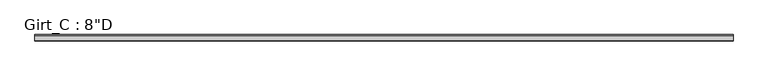
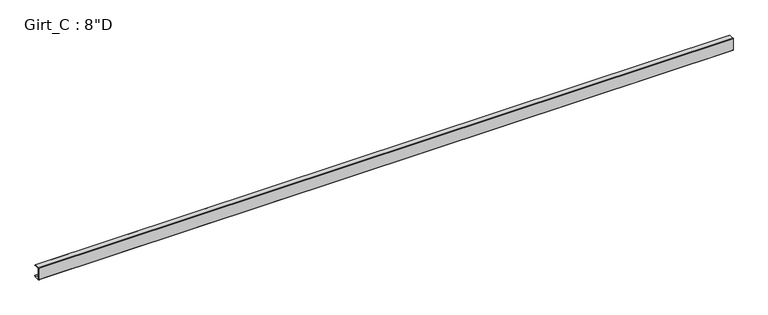
"""IFC4 building model written with IfcOpenShell, lengths in millimetres: beam geometry."""

from ifc_helpers import new_model, si_unit, point, frame, frame_2d, origin, place, context, project, spatial, polyline, circle_curve, trimmed, segment, composite_curve, outline, extrude, source, transform, mapped, element, save


def beam_dcccd556(model_context):
    return source(origin(), model_context, "Body", "SweptSolid", [
        extrude(outline(composite_curve([segment(polyline([(87.5109375, 101.6), (99.7560415, 87.0068534), (97.6278742, 85.221109), (86.2154765, 98.821875), (3.3005807, 98.821875)]), True, "CONTINUOUS"), segment(trimmed(circle_curve(frame_2d((3.3741066, 96.8381931)), 1.9850441), [point((3.3005807, 98.821875))], [point((1.3890625, 96.8381931))], True, "CARTESIAN"), True, "CONTINUOUS"), segment(polyline([(1.3890625, 96.8381931), (1.3890625, -96.8389339)]), True, "CONTINUOUS"), segment(trimmed(circle_curve(frame_2d((3.3748024, -96.8389339)), 1.9857399), [point((1.3890625, -96.8389339))], [point((3.2694106, -98.821875))], True, "CARTESIAN"), True, "CONTINUOUS"), segment(polyline([(3.2694106, -98.821875), (86.2154765, -98.821875), (97.6510975, -85.1934327), (99.7792647, -86.979177), (87.5109375, -101.6), (3.3734375, -101.6)]), True, "CONTINUOUS"), segment(trimmed(circle_curve(frame_2d((3.3734375, -96.8375)), 4.7625), [point((3.3734375, -101.6))], [point((-1.3890625, -96.8375))], False, "CARTESIAN"), True, "CONTINUOUS"), segment(polyline([(-1.3890625, -96.8375), (-1.3890625, 96.8375)]), True, "CONTINUOUS"), segment(trimmed(circle_curve(frame_2d((3.3734375, 96.8375)), 4.7625), [point((-1.3890625, 96.8375))], [point((3.3734375, 101.6))], False, "CARTESIAN"), True, "CONTINUOUS"), segment(polyline([(3.3734375, 101.6), (87.5109375, 101.6)]), True, "CONTINUOUS")], self_intersect=False)), frame((-5575.3, 0.0, 0.0), z_axis=(1.0, 0.0, 0.0), x_axis=(0.0, 1.0, 0.0)), (0.0, 0.0, 1.0), 11150.6),
    ])


if __name__ == "__main__":
    model = new_model("IFC4")
    model_context = context("Model", 3, world=origin())
    ifc_project = project(units=[si_unit("LENGTHUNIT", "METRE", prefix="MILLI")], contexts=[model_context])
    site = spatial("IfcSite", under=ifc_project)
    building = spatial("IfcBuilding", under=site)
    placement = place(None, origin())
    beam_shape = beam_dcccd556(model_context)
    element("IfcBeam", 1, ObjectType="Girt_C : 8\"D", at=placement, inside=building, context=model_context, shape_type="MappedRepresentation", body=[
        mapped(beam_shape, transform((0.0, 0.0, 0.0), x_axis=(1.0, 0.0, 0.0), y_axis=(0.0, 1.0, 0.0), z_axis=(0.0, 0.0, 1.0))),
    ])
    save(model, "model.ifc")

# Revit data of these elements
# Type "Girt_C : 8\"D"
#   half leg = 0' - 1 3/4"
#   Web_Thickness = 0' - 0 7/64"
#   Length [instance default] = 10' - 0"
#   Leg_1 = 0' - 3 1/2"
#   Height = 0' - 8"
#   Structural Material [instance default] = none
# Element 1 (IfcBeam, "Girt_C : 8\"D")
#   Structural Material = GALVANIZED 'CEE' SECTION (8.0x3.5C - SEE STRUCT. DWGS)
#   Materials on its faces: "GALVANIZED 'CEE' SECTION (8.0x3.5C - SEE STRUCT. DWGS)"
# Materials
#   "GALVANIZED 'CEE' SECTION (8.0x3.5C - SEE STRUCT. DWGS)": class "Metal", colour RGB 137 146 153, transparency 0, Description = "Steel, mill finish", Cost = 0
